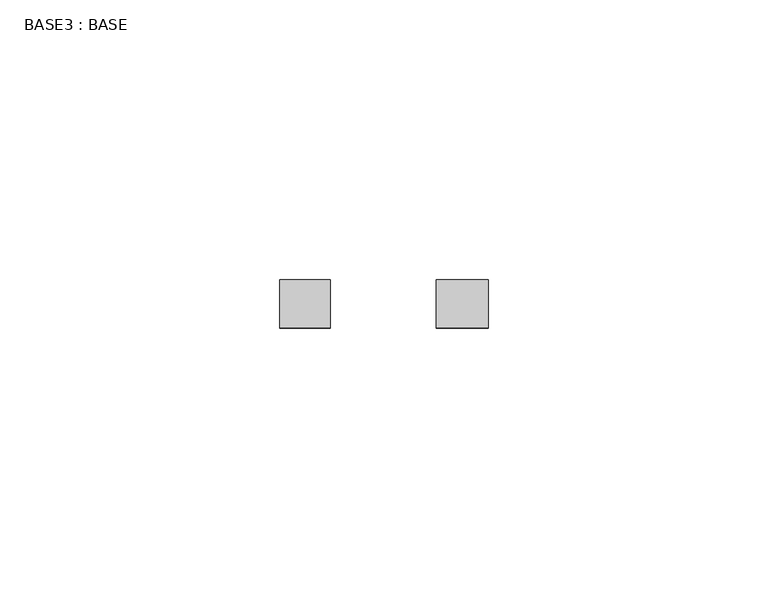
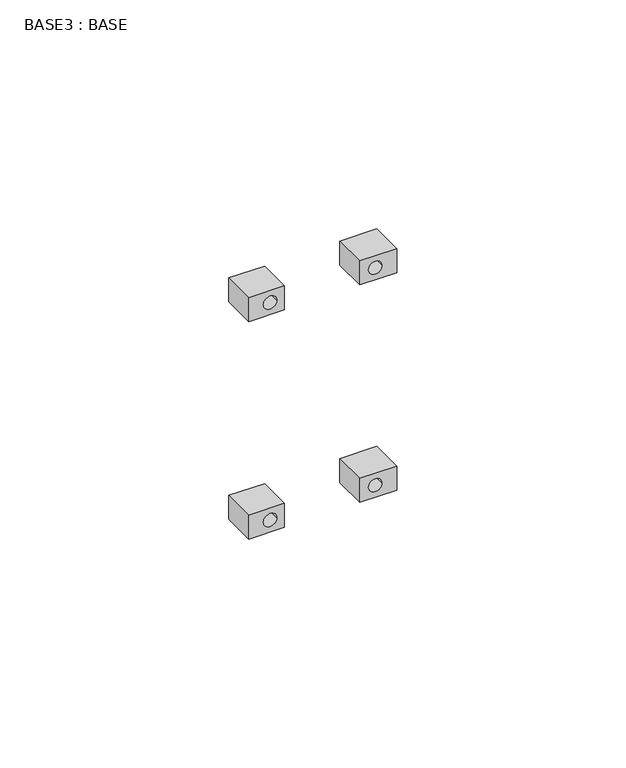
"""IFC4 building model written with IfcOpenShell, lengths in millimetres: proxy geometry, BASE3 : BASE."""

import ifcopenshell
import ifcopenshell.guid

model = None  # the IFC model being written
_history = None  # IfcOwnerHistory: only IFC2X3 demands one
_inside = {}  # id of a spatial element -> (the spatial element, [elements in it])
_under = {}  # id of a project, library or spatial element -> (it, [spatial elements below it])
_declared = {}  # id of a project -> (the project, [libraries it declares])
_typed = {}  # id of a type object -> (the type object, [elements of that type])
_made_of = {}  # id of a material, layer set ... -> (it, [elements and type objects made of it])


def new_model(schema):
    """Start an empty IFC model of exactly this schema.

    Asked for "IFC4X3", IfcOpenShell would pick the latest addendum, in which some entities
    have other attributes; the version numbers below select the first issue.
    IFC2X3 requires an IfcOwnerHistory on every rooted entity: one is made here for all.
    """
    global model, _history
    if schema == "IFC4X3":
        model = ifcopenshell.file(schema_version=(4, 3, 0, 0))
    else:
        model = ifcopenshell.file(schema=schema)
    _inside.clear()
    _under.clear()
    _declared.clear()
    _typed.clear()
    _made_of.clear()
    _history = None
    if model.schema == "IFC2X3":
        org = make("IfcOrganization", Name="unknown")
        user = make(
            "IfcPersonAndOrganization",
            ThePerson=make("IfcPerson", FamilyName="unknown"),
            TheOrganization=org,
        )
        app = make(
            "IfcApplication",
            ApplicationDeveloper=org,
            Version="unknown",
            ApplicationFullName="unknown",
            ApplicationIdentifier="unknown",
        )
        _history = make(
            "IfcOwnerHistory",
            OwningUser=user,
            OwningApplication=app,
            ChangeAction="ADDED",
            CreationDate=0,
        )
    return model


def make(cls, **values):
    """One entity of the class cls with the attributes given. An attribute that is None is left unset."""
    return model.create_entity(
        cls, **{name: value for name, value in values.items() if value is not None}
    )


def rooted(cls, **values):
    """An entity with a GlobalId (a new one), such as an element, a storey or a relation."""
    return make(cls, GlobalId=ifcopenshell.guid.new(), OwnerHistory=_history, **values)


def si_unit(unit_type, name, prefix=None):
    """IfcSIUnit, for example si_unit("LENGTHUNIT", "METRE", prefix="MILLI")."""
    return make("IfcSIUnit", UnitType=unit_type, Prefix=prefix, Name=name)


def assignment(units):
    """IfcUnitAssignment: the units of a project."""
    return None if units is None else make("IfcUnitAssignment", Units=units)


def point(xyz):
    """IfcCartesianPoint."""
    return None if xyz is None else make("IfcCartesianPoint", Coordinates=xyz)


def direction(xyz):
    """IfcDirection."""
    return None if xyz is None else make("IfcDirection", DirectionRatios=xyz)


def frame(location, z_axis=None, x_axis=None):
    """IfcAxis2Placement3D, a coordinate frame: its origin and axes. An axis left out is left unset."""
    return make(
        "IfcAxis2Placement3D",
        Location=point(location),
        Axis=direction(z_axis),
        RefDirection=direction(x_axis),
    )


def frame_2d(location, x_axis=None):
    """IfcAxis2Placement2D, a coordinate frame in the plane: its origin and x axis."""
    return make(
        "IfcAxis2Placement2D", Location=point(location), RefDirection=direction(x_axis)
    )


def origin():
    """The frame at (0, 0, 0) with its axes left unset."""
    return frame((0.0, 0.0, 0.0))


def place(relative_to, where):
    """IfcLocalPlacement: puts the frame where relative to a parent placement (None: the world)."""
    return make(
        "IfcLocalPlacement", PlacementRelTo=relative_to, RelativePlacement=where
    )


def context(
    kind, dimensions, precision=None, world=None, true_north=None, identifier=None
):
    """IfcGeometricRepresentationContext, for example the 3D "Model" context."""
    return make(
        "IfcGeometricRepresentationContext",
        ContextIdentifier=identifier,
        ContextType=kind,
        CoordinateSpaceDimension=dimensions,
        Precision=precision,
        WorldCoordinateSystem=world,
        TrueNorth=true_north,
    )


def project(units=None, contexts=None):
    """IfcProject with its units and contexts."""
    return rooted(
        "IfcProject",
        Name="project",
        RepresentationContexts=contexts,
        UnitsInContext=assignment(units),
    )


def spatial(cls, under=None, at=None, **own):
    """A site, building, storey or space (cls), placed at a placement, below another one or the project."""
    s = rooted(cls, ObjectPlacement=at, **own)
    if under is not None:
        _under.setdefault(under.id(), (under, []))[1].append(s)
    return s


def polyline(points):
    """IfcPolyline through the points."""
    return make("IfcPolyline", Points=[point(p) for p in points])


def circle_curve(where, radius):
    """IfcCircle in the frame where."""
    return make("IfcCircle", Position=where, Radius=radius)


def trimmed(basis, trim1, trim2, sense, master):
    """IfcTrimmedCurve: the piece of a basis curve between two trims."""
    return make(
        "IfcTrimmedCurve",
        BasisCurve=basis,
        Trim1=trim1,
        Trim2=trim2,
        SenseAgreement=sense,
        MasterRepresentation=master,
    )


def segment(curve, same_sense, transition):
    """IfcCompositeCurveSegment."""
    return make(
        "IfcCompositeCurveSegment",
        Transition=transition,
        SameSense=same_sense,
        ParentCurve=curve,
    )


def composite_curve(segments, self_intersect=None):
    """IfcCompositeCurve: segments joined end to end."""
    return make("IfcCompositeCurve", Segments=segments, SelfIntersect=self_intersect)


def outline(outer, holes=None, kind="AREA"):
    """IfcArbitraryClosedProfileDef: a profile drawn as a closed curve; with holes, ...WithVoids."""
    if holes is None:
        return make("IfcArbitraryClosedProfileDef", ProfileType=kind, OuterCurve=outer)
    return make(
        "IfcArbitraryProfileDefWithVoids",
        ProfileType=kind,
        OuterCurve=outer,
        InnerCurves=holes,
    )


def extrude(swept, where, along, depth):
    """IfcExtrudedAreaSolid: the profile swept, set in the frame where, extruded along a direction by depth."""
    return make(
        "IfcExtrudedAreaSolid",
        SweptArea=swept,
        Position=where,
        ExtrudedDirection=direction(along),
        Depth=depth,
    )


def shape(context_of_items, identifier, shape_type, items):
    """IfcShapeRepresentation: the items that make up one representation, for example the "Body"."""
    return make(
        "IfcShapeRepresentation",
        ContextOfItems=context_of_items,
        RepresentationIdentifier=identifier,
        RepresentationType=shape_type,
        Items=items,
    )


def source(mapping_origin, context_of_items, identifier, shape_type, items):
    """IfcRepresentationMap: a shape defined once, which mapped items show again and again."""
    return make(
        "IfcRepresentationMap",
        MappingOrigin=mapping_origin,
        MappedRepresentation=shape(context_of_items, identifier, shape_type, items),
    )


def transform(
    local_origin,
    x_axis=None,
    y_axis=None,
    z_axis=None,
    scale=None,
    scale2=None,
    scale3=None,
    uniform=True,
):
    """IfcCartesianTransformationOperator3D, or its non-uniform kind. x_axis, y_axis, z_axis: its Axis1, 2, 3."""
    if uniform:
        return make(
            "IfcCartesianTransformationOperator3D",
            Axis1=direction(x_axis),
            Axis2=direction(y_axis),
            LocalOrigin=point(local_origin),
            Scale=scale,
            Axis3=direction(z_axis),
        )
    return make(
        "IfcCartesianTransformationOperator3DnonUniform",
        Axis1=direction(x_axis),
        Axis2=direction(y_axis),
        LocalOrigin=point(local_origin),
        Scale=scale,
        Axis3=direction(z_axis),
        Scale2=scale2,
        Scale3=scale3,
    )


def mapped(mapping_source, mapping_target):
    """IfcMappedItem: shows the shape of a source again, moved by a transform."""
    return make(
        "IfcMappedItem", MappingSource=mapping_source, MappingTarget=mapping_target
    )


def made_of(thing, what):
    """Note that an element or type object is made of a material, layer set ...; save() writes the relation."""
    if what is not None:
        _made_of.setdefault(what.id(), (what, []))[1].append(thing)
    return thing


def element(
    cls,
    number,
    at=None,
    inside=None,
    cuts=None,
    type_object=None,
    material=None,
    context=None,
    identifier="Body",
    shape_type=None,
    held_by="IfcProductDefinitionShape",
    body=None,
    shapes=None,
    **own,
):
    """One element of the class cls, such as IfcWall. Its Tag is "e" and its number.

    at: its placement. inside: the storey or other place that contains it. cuts: it is an
    opening in that element (IfcRelVoidsElement). A single representation is given by context,
    identifier, shape_type and body (its items); several are given by shapes. held_by: the class
    of the entity that holds the representations. save() writes the other relations.
    """
    e = rooted(cls, Tag="e%d" % number, ObjectPlacement=at, **own)
    if body is not None:
        shapes = [shape(context, identifier, shape_type, body)]
    if shapes is not None:
        e.Representation = make(held_by, Representations=shapes)
    if inside is not None:
        _inside.setdefault(inside.id(), (inside, []))[1].append(e)
    if cuts is not None:
        rooted(
            "IfcRelVoidsElement", RelatingBuildingElement=cuts, RelatedOpeningElement=e
        )
    if type_object is not None:
        _typed.setdefault(type_object.id(), (type_object, []))[1].append(e)
    return made_of(e, material)


def aggregate(whole, parts):
    """IfcRelAggregates: a whole, such as a stair, and the parts it consists of."""
    return rooted("IfcRelAggregates", RelatingObject=whole, RelatedObjects=parts)


def save(model, path):
    """Write the relations noted so far, then the file.

    IfcRelAggregates (storeys below a building ...), IfcRelContainedInSpatialStructure (elements
    in a storey), IfcRelDefinesByType, IfcRelAssociatesMaterial and IfcRelDeclares: one each for
    every whole, place, type object, material and project.
    """
    for whole, parts in _under.values():
        aggregate(whole, parts)
    for where, things in _inside.values():
        rooted(
            "IfcRelContainedInSpatialStructure",
            RelatedElements=things,
            RelatingStructure=where,
        )
    for kind, things in _typed.values():
        rooted("IfcRelDefinesByType", RelatedObjects=things, RelatingType=kind)
    for what, things in _made_of.values():
        rooted("IfcRelAssociatesMaterial", RelatedObjects=things, RelatingMaterial=what)
    for by, libraries in _declared.values():
        rooted("IfcRelDeclares", RelatingContext=by, RelatedDefinitions=libraries)
    model.write(path)


def base3_base_5e775e04(model_context):
    return source(origin(), model_context, "Body", "SweptSolid", [
        extrude(outline(polyline([(59.8, 2465.0719295), (59.8, 2474.3719295), (66.2, 2474.3719295), (66.2, 2465.0719295), (59.8, 2465.0719295)]), holes=[composite_curve([segment(trimmed(circle_curve(frame_2d((63.0, 2468.9719295)), 1.7), [point((63.0, 2467.2719295))], [point((63.0, 2470.6719295))], True, "CARTESIAN"), True, "CONTINUOUS"), segment(trimmed(circle_curve(frame_2d((63.0, 2468.9719295)), 1.7), [point((63.0, 2470.6719295))], [point((63.0, 2467.2719295))], True, "CARTESIAN"), True, "CONTINUOUS")], self_intersect=False)]), frame((0.0, 1296.9192449, 0.0), z_axis=(0.0, 1.0, 0.0), x_axis=(0.0, 0.0, 1.0)), (0.0, 0.0, 1.0), 8.6306009),
        extrude(outline(polyline([(59.8, 2437.0719295), (59.8, 2446.0719295), (66.2, 2446.0719295), (66.2, 2437.0719295), (59.8, 2437.0719295)]), holes=[composite_curve([segment(trimmed(circle_curve(frame_2d((63.0, 2442.4719295)), 1.7), [point((63.0, 2444.1719295))], [point((63.0, 2440.7719295))], True, "CARTESIAN"), True, "CONTINUOUS"), segment(trimmed(circle_curve(frame_2d((63.0, 2442.4719295)), 1.7), [point((63.0, 2440.7719295))], [point((63.0, 2444.1719295))], True, "CARTESIAN"), True, "CONTINUOUS")], self_intersect=False)]), frame((0.0, 1296.9192449, 0.0), z_axis=(0.0, 1.0, 0.0), x_axis=(0.0, 0.0, 1.0)), (0.0, 0.0, 1.0), 8.6306009),
        extrude(outline(polyline([(1.8, 2465.0719295), (1.8, 2474.3719295), (8.2, 2474.3719295), (8.2, 2465.0719295), (1.8, 2465.0719295)]), holes=[composite_curve([segment(trimmed(circle_curve(frame_2d((5.0, 2468.9719295)), 1.7), [point((5.0, 2470.6719295))], [point((5.0, 2467.2719295))], True, "CARTESIAN"), True, "CONTINUOUS"), segment(trimmed(circle_curve(frame_2d((5.0, 2468.9719295)), 1.7), [point((5.0, 2467.2719295))], [point((5.0, 2470.6719295))], True, "CARTESIAN"), True, "CONTINUOUS")], self_intersect=False)]), frame((0.0, 1296.9192449, 0.0), z_axis=(0.0, 1.0, 0.0), x_axis=(0.0, 0.0, 1.0)), (0.0, 0.0, 1.0), 8.6306009),
        extrude(outline(polyline([(1.8, 2446.0719295), (8.2, 2446.0719295), (8.2, 2437.0719295), (1.8, 2437.0719295), (1.8, 2446.0719295)]), holes=[composite_curve([segment(trimmed(circle_curve(frame_2d((5.0, 2442.4719295)), 1.7), [point((5.0, 2444.1719295))], [point((5.0, 2440.7719295))], True, "CARTESIAN"), True, "CONTINUOUS"), segment(trimmed(circle_curve(frame_2d((5.0, 2442.4719295)), 1.7), [point((5.0, 2440.7719295))], [point((5.0, 2444.1719295))], True, "CARTESIAN"), True, "CONTINUOUS")], self_intersect=False)]), frame((0.0, 1296.9192449, 0.0), z_axis=(0.0, 1.0, 0.0), x_axis=(0.0, 0.0, 1.0)), (0.0, 0.0, 1.0), 8.6306009),
    ])


if __name__ == "__main__":
    model = new_model("IFC4")
    model_context = context("Model", 3, world=origin())
    ifc_project = project(units=[si_unit("LENGTHUNIT", "METRE", prefix="MILLI")], contexts=[model_context])
    site = spatial("IfcSite", under=ifc_project)
    building = spatial("IfcBuilding", under=site)
    placement = place(None, origin())
    base3_base_shape = base3_base_5e775e04(model_context)
    element("IfcBuildingElementProxy", 1, Name="BASE3 : BASE", ObjectType="BASE3 : BASE", at=placement, inside=building, context=model_context, shape_type="MappedRepresentation", body=[
        mapped(base3_base_shape, transform((0.0, 0.0, 0.0), x_axis=(1.0, 0.0, 0.0), y_axis=(0.0, 1.0, 0.0), z_axis=(0.0, 0.0, 1.0))),
    ])
    save(model, "model.ifc")

# Revit data of these elements
# Project information
#   Data de emissão do projeto = "Data de emissão"
#   Status do projeto = "Status do projeto"
#   Nome do cliente = "Proprietário"
#   Endereço do projeto = "Insira aqui o endereço"
#   Nome do projeto = "Nome do projeto"
#   Número do projeto = "0001"
# Element 1 (IfcBuildingElementProxy, "BASE3 : BASE")
#   Materials on its faces: ".BOX FUNDO"
# Materials
#   ".BOX FUNDO": class "Vidro", colour RGB 236 240 239, transparency 0.15, Cost = 0
